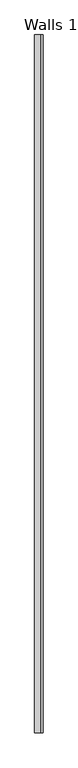
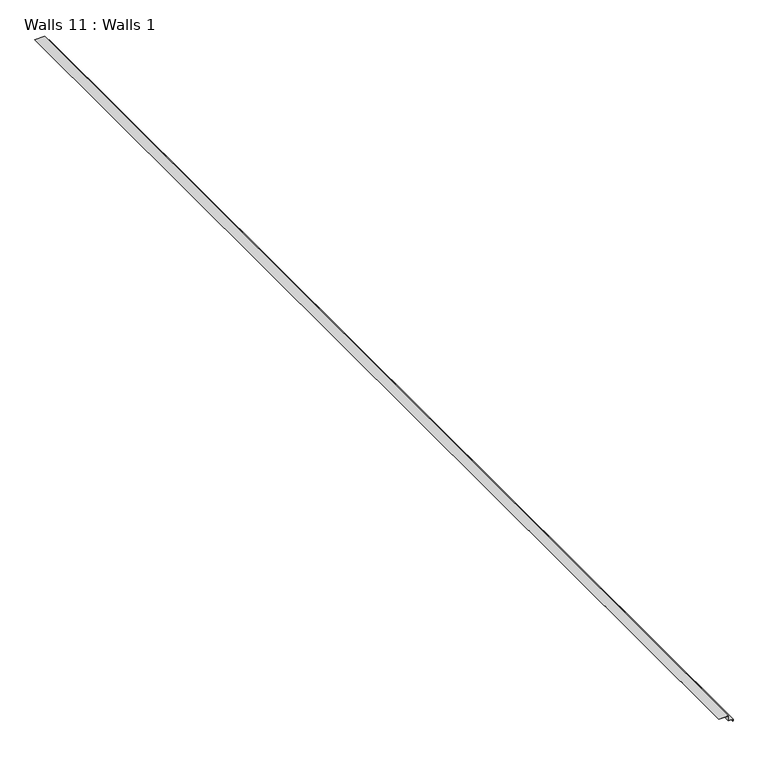
"""IFC4 building model written with IfcOpenShell, lengths in millimetres: proxy geometry, Walls 11 : Walls 1."""

from ifc_helpers import new_model, si_unit, frame, origin, place, context, project, spatial, polyline, outline, extrude, source, transform, mapped, element, save


def walls_11_walls_1_9dd18fde(model_context):
    return source(origin(), model_context, "Body", "SweptSolid", [
        extrude(outline(polyline([(269367.1879188, 32076.6247028), (269367.1879188, 32165.7744875), (269318.6806603, 32165.7744875), (269318.6806603, 32209.9472589), (269302.266899, 32209.9472589), (269302.266899, 32211.5347589), (269320.2681603, 32211.5347589), (269320.2681603, 32167.3619875), (269368.7754188, 32167.3619875), (269368.7754188, 32076.6247028), (269367.1879188, 32076.6247028)])), frame((0.0, 29659.1292286, 0.0), z_axis=(0.0, 1.0, 0.0), x_axis=(0.0, 0.0, 1.0)), (0.0, 0.0, 1.0), 11114.5564326),
    ])


if __name__ == "__main__":
    model = new_model("IFC4")
    model_context = context("Model", 3, world=origin())
    ifc_project = project(units=[si_unit("LENGTHUNIT", "METRE", prefix="MILLI")], contexts=[model_context])
    site = spatial("IfcSite", under=ifc_project)
    building = spatial("IfcBuilding", under=site)
    placement = place(None, origin())
    walls_11_walls_1_shape = walls_11_walls_1_9dd18fde(model_context)
    element("IfcBuildingElementProxy", 1, Name="Walls 11 : Walls 1", ObjectType="Walls 11 : Walls 1", at=placement, inside=building, context=model_context, shape_type="MappedRepresentation", body=[
        mapped(walls_11_walls_1_shape, transform((0.0, 0.0, 0.0), x_axis=(1.0, 0.0, 0.0), y_axis=(0.0, 1.0, 0.0), z_axis=(0.0, 0.0, 1.0))),
    ])
    save(model, "model.ifc")

# Revit data of these elements
# Element 1 (IfcBuildingElementProxy, "Walls 11 : Walls 1")
#   Materials on its faces: "GALV. BRAKE METAL - (COLOR: MATCH ALUM. WINDOWS)"
# Materials
#   "GALV. BRAKE METAL - (COLOR: MATCH ALUM. WINDOWS)": class "Generic", colour RGB 234 234 234, transparency 0, Cost = 0
